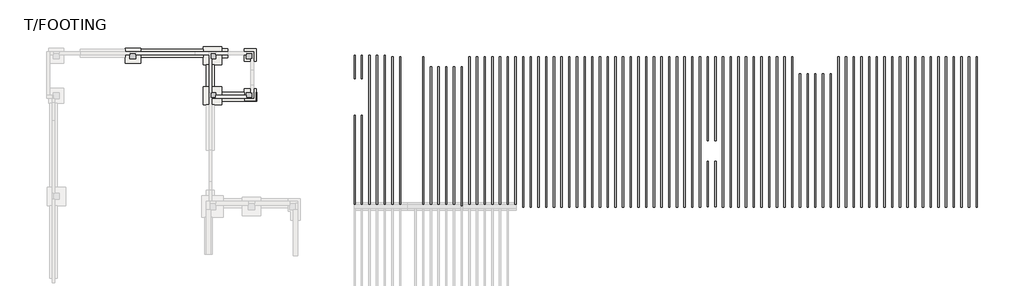
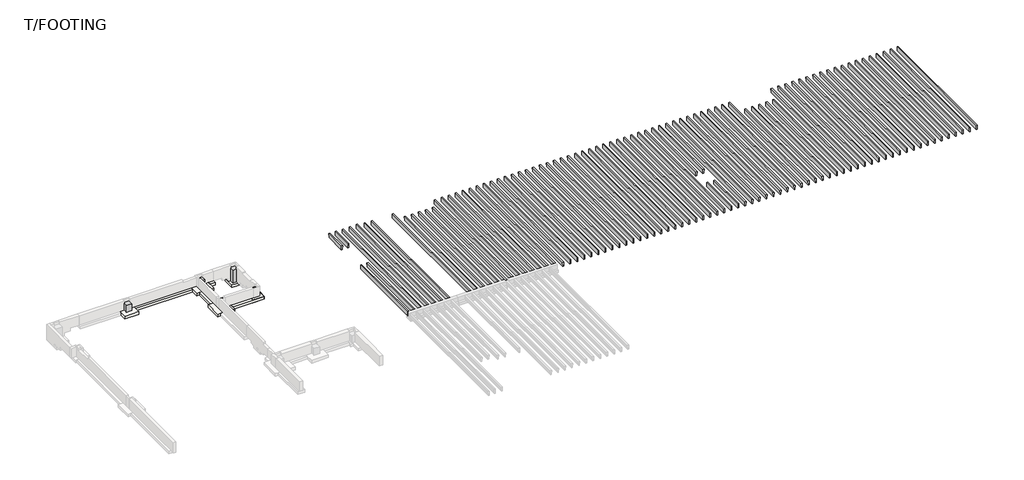
# One storey, part 3 of 3: 84 beams, 5 columns, 5 slabs, 4 footings.
"""IFC4 building model written with IfcOpenShell, lengths in millimetres."""

import ifcopenshell
import ifcopenshell.guid

model = None  # the IFC model being written
_history = None  # IfcOwnerHistory: only IFC2X3 demands one
_inside = {}  # id of a spatial element -> (the spatial element, [elements in it])
_under = {}  # id of a project, library or spatial element -> (it, [spatial elements below it])
_declared = {}  # id of a project -> (the project, [libraries it declares])
_typed = {}  # id of a type object -> (the type object, [elements of that type])
_made_of = {}  # id of a material, layer set ... -> (it, [elements and type objects made of it])


def new_model(schema):
    """Start an empty IFC model of exactly this schema.

    Asked for "IFC4X3", IfcOpenShell would pick the latest addendum, in which some entities
    have other attributes; the version numbers below select the first issue.
    IFC2X3 requires an IfcOwnerHistory on every rooted entity: one is made here for all.
    """
    global model, _history
    if schema == "IFC4X3":
        model = ifcopenshell.file(schema_version=(4, 3, 0, 0))
    else:
        model = ifcopenshell.file(schema=schema)
    _inside.clear()
    _under.clear()
    _declared.clear()
    _typed.clear()
    _made_of.clear()
    _history = None
    if model.schema == "IFC2X3":
        org = make("IfcOrganization", Name="unknown")
        user = make(
            "IfcPersonAndOrganization",
            ThePerson=make("IfcPerson", FamilyName="unknown"),
            TheOrganization=org,
        )
        app = make(
            "IfcApplication",
            ApplicationDeveloper=org,
            Version="unknown",
            ApplicationFullName="unknown",
            ApplicationIdentifier="unknown",
        )
        _history = make(
            "IfcOwnerHistory",
            OwningUser=user,
            OwningApplication=app,
            ChangeAction="ADDED",
            CreationDate=0,
        )
    return model


def make(cls, **values):
    """One entity of the class cls with the attributes given. An attribute that is None is left unset."""
    return model.create_entity(
        cls, **{name: value for name, value in values.items() if value is not None}
    )


def rooted(cls, **values):
    """An entity with a GlobalId (a new one), such as an element, a storey or a relation."""
    return make(cls, GlobalId=ifcopenshell.guid.new(), OwnerHistory=_history, **values)


def si_unit(unit_type, name, prefix=None):
    """IfcSIUnit, for example si_unit("LENGTHUNIT", "METRE", prefix="MILLI")."""
    return make("IfcSIUnit", UnitType=unit_type, Prefix=prefix, Name=name)


def assignment(units):
    """IfcUnitAssignment: the units of a project."""
    return None if units is None else make("IfcUnitAssignment", Units=units)


def point(xyz):
    """IfcCartesianPoint."""
    return None if xyz is None else make("IfcCartesianPoint", Coordinates=xyz)


def direction(xyz):
    """IfcDirection."""
    return None if xyz is None else make("IfcDirection", DirectionRatios=xyz)


def frame(location, z_axis=None, x_axis=None):
    """IfcAxis2Placement3D, a coordinate frame: its origin and axes. An axis left out is left unset."""
    return make(
        "IfcAxis2Placement3D",
        Location=point(location),
        Axis=direction(z_axis),
        RefDirection=direction(x_axis),
    )


def origin():
    """The frame at (0, 0, 0) with its axes left unset."""
    return frame((0.0, 0.0, 0.0))


def place(relative_to, where):
    """IfcLocalPlacement: puts the frame where relative to a parent placement (None: the world)."""
    return make(
        "IfcLocalPlacement", PlacementRelTo=relative_to, RelativePlacement=where
    )


def context(
    kind, dimensions, precision=None, world=None, true_north=None, identifier=None
):
    """IfcGeometricRepresentationContext, for example the 3D "Model" context."""
    return make(
        "IfcGeometricRepresentationContext",
        ContextIdentifier=identifier,
        ContextType=kind,
        CoordinateSpaceDimension=dimensions,
        Precision=precision,
        WorldCoordinateSystem=world,
        TrueNorth=true_north,
    )


def project(units=None, contexts=None):
    """IfcProject with its units and contexts."""
    return rooted(
        "IfcProject",
        Name="project",
        RepresentationContexts=contexts,
        UnitsInContext=assignment(units),
    )


def spatial(cls, under=None, at=None, **own):
    """A site, building, storey or space (cls), placed at a placement, below another one or the project."""
    s = rooted(cls, ObjectPlacement=at, **own)
    if under is not None:
        _under.setdefault(under.id(), (under, []))[1].append(s)
    return s


def polyline(points):
    """IfcPolyline through the points."""
    return make("IfcPolyline", Points=[point(p) for p in points])


def outline(outer, holes=None, kind="AREA"):
    """IfcArbitraryClosedProfileDef: a profile drawn as a closed curve; with holes, ...WithVoids."""
    if holes is None:
        return make("IfcArbitraryClosedProfileDef", ProfileType=kind, OuterCurve=outer)
    return make(
        "IfcArbitraryProfileDefWithVoids",
        ProfileType=kind,
        OuterCurve=outer,
        InnerCurves=holes,
    )


def extrude(swept, where, along, depth):
    """IfcExtrudedAreaSolid: the profile swept, set in the frame where, extruded along a direction by depth."""
    return make(
        "IfcExtrudedAreaSolid",
        SweptArea=swept,
        Position=where,
        ExtrudedDirection=direction(along),
        Depth=depth,
    )


def faces_of(points, faces, orient=None, outer=None):
    """IfcFace entities. A face is a list of loops; a loop is a list of indices into points, from 0.

    orient and outer hold one flag for each loop. By default every Orientation is true, the
    first loop of a face is its IfcFaceOuterBound and the others are IfcFaceBound.
    """
    made = []
    for i, loops in enumerate(faces):
        bounds = []
        for j, loop in enumerate(loops):
            is_outer = j == 0 if outer is None else outer[i][j]
            bounds.append(
                make(
                    "IfcFaceOuterBound" if is_outer else "IfcFaceBound",
                    Bound=make("IfcPolyLoop", Polygon=[points[k] for k in loop]),
                    Orientation=True if orient is None else orient[i][j],
                )
            )
        made.append(make("IfcFace", Bounds=bounds))
    return made


def faceted_brep(points, faces, orient=None, outer=None, voids=None):
    """IfcFacetedBrep: a solid bounded by flat faces; with voids (closed shells), ...WithVoids."""
    shared = [point(p) for p in points]
    hull = make("IfcClosedShell", CfsFaces=faces_of(shared, faces, orient, outer))
    if voids is None:
        return make("IfcFacetedBrep", Outer=hull)
    return make(
        "IfcFacetedBrepWithVoids",
        Outer=hull,
        Voids=[
            make(cls, CfsFaces=faces_of(shared, fs, o, b)) for cls, fs, o, b in voids
        ],
    )


def shape(context_of_items, identifier, shape_type, items):
    """IfcShapeRepresentation: the items that make up one representation, for example the "Body"."""
    return make(
        "IfcShapeRepresentation",
        ContextOfItems=context_of_items,
        RepresentationIdentifier=identifier,
        RepresentationType=shape_type,
        Items=items,
    )


def source(mapping_origin, context_of_items, identifier, shape_type, items):
    """IfcRepresentationMap: a shape defined once, which mapped items show again and again."""
    return make(
        "IfcRepresentationMap",
        MappingOrigin=mapping_origin,
        MappedRepresentation=shape(context_of_items, identifier, shape_type, items),
    )


def transform(
    local_origin,
    x_axis=None,
    y_axis=None,
    z_axis=None,
    scale=None,
    scale2=None,
    scale3=None,
    uniform=True,
):
    """IfcCartesianTransformationOperator3D, or its non-uniform kind. x_axis, y_axis, z_axis: its Axis1, 2, 3."""
    if uniform:
        return make(
            "IfcCartesianTransformationOperator3D",
            Axis1=direction(x_axis),
            Axis2=direction(y_axis),
            LocalOrigin=point(local_origin),
            Scale=scale,
            Axis3=direction(z_axis),
        )
    return make(
        "IfcCartesianTransformationOperator3DnonUniform",
        Axis1=direction(x_axis),
        Axis2=direction(y_axis),
        LocalOrigin=point(local_origin),
        Scale=scale,
        Axis3=direction(z_axis),
        Scale2=scale2,
        Scale3=scale3,
    )


def mapped(mapping_source, mapping_target):
    """IfcMappedItem: shows the shape of a source again, moved by a transform."""
    return make(
        "IfcMappedItem", MappingSource=mapping_source, MappingTarget=mapping_target
    )


def made_of(thing, what):
    """Note that an element or type object is made of a material, layer set ...; save() writes the relation."""
    if what is not None:
        _made_of.setdefault(what.id(), (what, []))[1].append(thing)
    return thing


def element(
    cls,
    number,
    at=None,
    inside=None,
    cuts=None,
    type_object=None,
    material=None,
    context=None,
    identifier="Body",
    shape_type=None,
    held_by="IfcProductDefinitionShape",
    body=None,
    shapes=None,
    **own,
):
    """One element of the class cls, such as IfcWall. Its Tag is "e" and its number.

    at: its placement. inside: the storey or other place that contains it. cuts: it is an
    opening in that element (IfcRelVoidsElement). A single representation is given by context,
    identifier, shape_type and body (its items); several are given by shapes. held_by: the class
    of the entity that holds the representations. save() writes the other relations.
    """
    e = rooted(cls, Tag="e%d" % number, ObjectPlacement=at, **own)
    if body is not None:
        shapes = [shape(context, identifier, shape_type, body)]
    if shapes is not None:
        e.Representation = make(held_by, Representations=shapes)
    if inside is not None:
        _inside.setdefault(inside.id(), (inside, []))[1].append(e)
    if cuts is not None:
        rooted(
            "IfcRelVoidsElement", RelatingBuildingElement=cuts, RelatedOpeningElement=e
        )
    if type_object is not None:
        _typed.setdefault(type_object.id(), (type_object, []))[1].append(e)
    return made_of(e, material)


def aggregate(whole, parts):
    """IfcRelAggregates: a whole, such as a stair, and the parts it consists of."""
    return rooted("IfcRelAggregates", RelatingObject=whole, RelatedObjects=parts)


def save(model, path):
    """Write the relations noted so far, then the file.

    IfcRelAggregates (storeys below a building ...), IfcRelContainedInSpatialStructure (elements
    in a storey), IfcRelDefinesByType, IfcRelAssociatesMaterial and IfcRelDeclares: one each for
    every whole, place, type object, material and project.
    """
    for whole, parts in _under.values():
        aggregate(whole, parts)
    for where, things in _inside.values():
        rooted(
            "IfcRelContainedInSpatialStructure",
            RelatedElements=things,
            RelatingStructure=where,
        )
    for kind, things in _typed.values():
        rooted("IfcRelDefinesByType", RelatedObjects=things, RelatingType=kind)
    for what, things in _made_of.values():
        rooted("IfcRelAssociatesMaterial", RelatedObjects=things, RelatingMaterial=what)
    for by, libraries in _declared.values():
        rooted("IfcRelDeclares", RelatingContext=by, RelatedDefinitions=libraries)
    model.write(path)


def precast_cone_shaped_beam_double_t_5f2c7775(model_context):
    return source(origin(), model_context, "Body", "SweptSolid", [
        extrude(outline(polyline([(50.8, -228.6), (-50.8, -228.6), (-63.5, 228.6), (63.5, 228.6), (50.8, -228.6)])), frame((-7353.3, 0.0, 0.0), z_axis=(1.0, 0.0, 0.0), x_axis=(0.0, 1.0, 0.0)), (0.0, 0.0, 1.0), 14693.9),
    ])


def precast_cone_shaped_beam_double_t_00600c4c(model_context):
    return source(origin(), model_context, "Body", "SweptSolid", [
        extrude(outline(polyline([(50.8, -228.6), (-50.8, -228.6), (-63.5, 228.6), (63.5, 228.6), (50.8, -228.6)])), frame((-7556.5, 0.0, 0.0), z_axis=(1.0, 0.0, 0.0), x_axis=(0.0, 1.0, 0.0)), (0.0, 0.0, 1.0), 14897.1),
    ])


def precast_cone_shaped_beam_double_t_e3fa137c(model_context):
    return source(origin(), model_context, "Body", "SweptSolid", [
        extrude(outline(polyline([(50.8, -228.6), (-50.8, -228.6), (-63.5, 228.6), (63.5, 228.6), (50.8, -228.6)])), frame((-4296.56875, 0.0, 0.0), z_axis=(1.0, 0.0, 0.0), x_axis=(0.0, 1.0, 0.0)), (0.0, 0.0, 1.0), 8318.5),
    ])


def precast_cone_shaped_beam_double_t_ce46092e(model_context):
    return source(origin(), model_context, "Body", "SweptSolid", [
        extrude(outline(polyline([(-50.8, -228.6), (-63.5, 228.6), (63.5, 228.6), (50.8, -228.6), (-50.8, -228.6)])), frame((-2302.66875, 0.0, 0.0), z_axis=(1.0, 0.0, 0.0), x_axis=(0.0, 1.0, 0.0)), (0.0, 0.0, 1.0), 4495.8),
    ])


def precast_cone_shaped_beam_double_t_099a914b(model_context):
    return source(origin(), model_context, "Body", "SweptSolid", [
        extrude(outline(polyline([(50.8, -228.6), (-50.8, -228.6), (-63.5, 228.6), (63.5, 228.6), (50.8, -228.6)])), frame((-6574.63125, 0.0, 0.0), z_axis=(1.0, 0.0, 0.0), x_axis=(0.0, 1.0, 0.0)), (0.0, 0.0, 1.0), 13208.0),
    ])


def precast_cone_shaped_beam_double_t_b8a3e37e(model_context):
    return source(origin(), model_context, "Body", "SweptSolid", [
        extrude(outline(polyline([(50.8, -228.6), (-50.8, -228.6), (-63.5, 228.6), (63.5, 228.6), (50.8, -228.6)])), frame((-6727.03125, 0.0, 0.0), z_axis=(1.0, 0.0, 0.0), x_axis=(0.0, 1.0, 0.0)), (0.0, 0.0, 1.0), 13716.0),
    ])


def precast_cone_shaped_beam_double_t_383d5be5(model_context):
    return source(origin(), model_context, "Body", "SweptSolid", [
        extrude(outline(polyline([(50.8, -228.6), (-50.8, -228.6), (-63.5, 228.6), (63.5, 228.6), (50.8, -228.6)])), frame((-6930.23125, 0.0, 0.0), z_axis=(1.0, 0.0, 0.0), x_axis=(0.0, 1.0, 0.0)), (0.0, 0.0, 1.0), 13919.2),
    ])


def precast_cone_shaped_beam_double_t_e38496ef(model_context):
    return source(origin(), model_context, "Body", "SweptSolid", [
        extrude(outline(polyline([(50.8, -228.6), (-50.8, -228.6), (-63.5, 228.6), (63.5, 228.6), (50.8, -228.6)])), frame((-4311.8111314, 0.0, 0.0), z_axis=(1.0, 0.0, 0.0), x_axis=(0.0, 1.0, 0.0)), (0.0, 0.0, 1.0), 8885.5597628),
    ])


def precast_cone_shaped_beam_double_t_7663fcfe(model_context):
    return source(origin(), model_context, "Body", "SweptSolid", [
        extrude(outline(polyline([(-50.8, -228.6), (-63.5, 228.6), (63.5, 228.6), (50.8, -228.6), (-50.8, -228.6)])), frame((-1119.0263686, 0.0, 0.0), z_axis=(1.0, 0.0, 0.0), x_axis=(0.0, 1.0, 0.0)), (0.0, 0.0, 1.0), 2347.5902372),
    ])


def precast_cone_shaped_beam_double_t_3d71fa44(model_context):
    return source(origin(), model_context, "Body", "SweptSolid", [
        extrude(outline(polyline([(50.8, -228.6), (-50.8, -228.6), (-63.5, 228.6), (63.5, 228.6), (50.8, -228.6)])), frame((-7353.3, 0.0, 0.0), z_axis=(1.0, 0.0, 0.0), x_axis=(0.0, 1.0, 0.0)), (0.0, 0.0, 1.0), 14859.0),
    ])


model = new_model("IFC4")

# Units and contexts
model_context = context("Model", 3, world=origin())
ifc_project = project(units=[si_unit("LENGTHUNIT", "METRE", prefix="MILLI")], contexts=[model_context])

# Site, building, storey
site = spatial("IfcSite", under=ifc_project)
building = spatial("IfcBuilding", under=site)
storey = spatial("IfcBuildingStorey", under=building, Name="T/FOOTING", Elevation=-1092.2)

# Beams
placement = place(None, origin())
precast_cone_shaped_beam_double_t_shape = precast_cone_shaped_beam_double_t_5f2c7775(model_context)
element("IfcBeam", 1, ObjectType="Precast-Cone Shaped Beam : DOUBLE_T", at=placement, inside=storey, context=model_context, shape_type="MappedRepresentation", body=[
    mapped(precast_cone_shaped_beam_double_t_shape, transform((-28033.5909443, 5341.6768471, -279.4), x_axis=(0.0, 1.0, 0.0), y_axis=(-1.0, 0.0, 0.0), z_axis=(0.0, 0.0, 1.0))),
])
element("IfcBeam", 2, ObjectType="Precast-Cone Shaped Beam : DOUBLE_T", at=placement, inside=storey, context=model_context, shape_type="MappedRepresentation", body=[
    mapped(precast_cone_shaped_beam_double_t_shape, transform((-23461.5909443, 5341.6768471, -279.4), x_axis=(0.0, 1.0, 0.0), y_axis=(-1.0, 0.0, 0.0), z_axis=(0.0, 0.0, 1.0))),
])
element("IfcBeam", 3, ObjectType="Precast-Cone Shaped Beam : DOUBLE_T", at=placement, inside=storey, context=model_context, shape_type="MappedRepresentation", body=[
    mapped(precast_cone_shaped_beam_double_t_shape, transform((-22699.5909443, 5341.6768471, -279.4), x_axis=(0.0, 1.0, 0.0), y_axis=(-1.0, 0.0, 0.0), z_axis=(0.0, 0.0, 1.0))),
])
element("IfcBeam", 4, ObjectType="Precast-Cone Shaped Beam : DOUBLE_T", at=placement, inside=storey, context=model_context, shape_type="MappedRepresentation", body=[
    mapped(precast_cone_shaped_beam_double_t_shape, transform((-21940.4905844, 5341.6768471, -279.4), x_axis=(0.0, 1.0, 0.0), y_axis=(-1.0, 0.0, 0.0), z_axis=(0.0, 0.0, 1.0))),
])
element("IfcBeam", 5, ObjectType="Precast-Cone Shaped Beam : DOUBLE_T", at=placement, inside=storey, context=model_context, shape_type="MappedRepresentation", body=[
    mapped(precast_cone_shaped_beam_double_t_shape, transform((-21179.5348789, 5341.6768471, -279.4), x_axis=(0.0, 1.0, 0.0), y_axis=(-1.0, 0.0, 0.0), z_axis=(0.0, 0.0, 1.0))),
])
element("IfcBeam", 6, ObjectType="Precast-Cone Shaped Beam : DOUBLE_T", at=placement, inside=storey, context=model_context, shape_type="MappedRepresentation", body=[
    mapped(precast_cone_shaped_beam_double_t_shape, transform((-20417.5348789, 5341.6768471, -279.4), x_axis=(0.0, 1.0, 0.0), y_axis=(-1.0, 0.0, 0.0), z_axis=(0.0, 0.0, 1.0))),
])
element("IfcBeam", 7, ObjectType="Precast-Cone Shaped Beam : DOUBLE_T", at=placement, inside=storey, context=model_context, shape_type="MappedRepresentation", body=[
    mapped(precast_cone_shaped_beam_double_t_shape, transform((-19655.5348789, 5341.6768471, -279.4), x_axis=(0.0, 1.0, 0.0), y_axis=(-1.0, 0.0, 0.0), z_axis=(0.0, 0.0, 1.0))),
])
element("IfcBeam", 8, ObjectType="Precast-Cone Shaped Beam : DOUBLE_T", at=placement, inside=storey, context=model_context, shape_type="MappedRepresentation", body=[
    mapped(precast_cone_shaped_beam_double_t_shape, transform((-18893.5348789, 5341.6768471, -279.4), x_axis=(0.0, 1.0, 0.0), y_axis=(-1.0, 0.0, 0.0), z_axis=(0.0, 0.0, 1.0))),
])
element("IfcBeam", 9, ObjectType="Precast-Cone Shaped Beam : DOUBLE_T", at=placement, inside=storey, context=model_context, shape_type="MappedRepresentation", body=[
    mapped(precast_cone_shaped_beam_double_t_shape, transform((-30319.5909443, 5341.6768471, -279.4), x_axis=(0.0, 1.0, 0.0), y_axis=(-1.0, 0.0, 0.0), z_axis=(0.0, 0.0, 1.0))),
])
element("IfcBeam", 10, ObjectType="Precast-Cone Shaped Beam : DOUBLE_T", at=placement, inside=storey, context=model_context, shape_type="MappedRepresentation", body=[
    mapped(precast_cone_shaped_beam_double_t_shape, transform((-31081.5909443, 5341.6768471, -279.4), x_axis=(0.0, 1.0, 0.0), y_axis=(-1.0, 0.0, 0.0), z_axis=(0.0, 0.0, 1.0))),
])
precast_cone_shaped_beam_double_t_2_shape = precast_cone_shaped_beam_double_t_00600c4c(model_context)
element("IfcBeam", 11, ObjectType="Precast-Cone Shaped Beam : DOUBLE_T", at=placement, inside=storey, context=model_context, shape_type="MappedRepresentation", body=[
    mapped(precast_cone_shaped_beam_double_t_2_shape, transform((-18131.5348789, 5341.6768471, -279.4), x_axis=(0.0, 1.0, 0.0), y_axis=(-1.0, 0.0, 0.0), z_axis=(0.0, 0.0, 1.0))),
])
element("IfcBeam", 12, ObjectType="Precast-Cone Shaped Beam : DOUBLE_T", at=placement, inside=storey, context=model_context, shape_type="MappedRepresentation", body=[
    mapped(precast_cone_shaped_beam_double_t_2_shape, transform((-17369.5348789, 5341.6768471, -279.4), x_axis=(0.0, 1.0, 0.0), y_axis=(-1.0, 0.0, 0.0), z_axis=(0.0, 0.0, 1.0))),
])
element("IfcBeam", 13, ObjectType="Precast-Cone Shaped Beam : DOUBLE_T", at=placement, inside=storey, context=model_context, shape_type="MappedRepresentation", body=[
    mapped(precast_cone_shaped_beam_double_t_2_shape, transform((-16607.5348789, 5341.6768471, -279.4), x_axis=(0.0, 1.0, 0.0), y_axis=(-1.0, 0.0, 0.0), z_axis=(0.0, 0.0, 1.0))),
])
element("IfcBeam", 14, ObjectType="Precast-Cone Shaped Beam : DOUBLE_T", at=placement, inside=storey, context=model_context, shape_type="MappedRepresentation", body=[
    mapped(precast_cone_shaped_beam_double_t_2_shape, transform((-15845.5348789, 5341.6768471, -279.4), x_axis=(0.0, 1.0, 0.0), y_axis=(-1.0, 0.0, 0.0), z_axis=(0.0, 0.0, 1.0))),
])
element("IfcBeam", 15, ObjectType="Precast-Cone Shaped Beam : DOUBLE_T", at=placement, inside=storey, context=model_context, shape_type="MappedRepresentation", body=[
    mapped(precast_cone_shaped_beam_double_t_2_shape, transform((-15083.5348789, 5341.6768471, -279.4), x_axis=(0.0, 1.0, 0.0), y_axis=(-1.0, 0.0, 0.0), z_axis=(0.0, 0.0, 1.0))),
])
element("IfcBeam", 16, ObjectType="Precast-Cone Shaped Beam : DOUBLE_T", at=placement, inside=storey, context=model_context, shape_type="MappedRepresentation", body=[
    mapped(precast_cone_shaped_beam_double_t_2_shape, transform((-14321.5348789, 5341.6768471, -279.4), x_axis=(0.0, 1.0, 0.0), y_axis=(-1.0, 0.0, 0.0), z_axis=(0.0, 0.0, 1.0))),
])
element("IfcBeam", 17, ObjectType="Precast-Cone Shaped Beam : DOUBLE_T", at=placement, inside=storey, context=model_context, shape_type="MappedRepresentation", body=[
    mapped(precast_cone_shaped_beam_double_t_2_shape, transform((-13559.5348789, 5341.6768471, -279.4), x_axis=(0.0, 1.0, 0.0), y_axis=(-1.0, 0.0, 0.0), z_axis=(0.0, 0.0, 1.0))),
])
element("IfcBeam", 18, ObjectType="Precast-Cone Shaped Beam : DOUBLE_T", at=placement, inside=storey, context=model_context, shape_type="MappedRepresentation", body=[
    mapped(precast_cone_shaped_beam_double_t_2_shape, transform((-12797.5348789, 5341.6768471, -279.4), x_axis=(0.0, 1.0, 0.0), y_axis=(-1.0, 0.0, 0.0), z_axis=(0.0, 0.0, 1.0))),
])
element("IfcBeam", 19, ObjectType="Precast-Cone Shaped Beam : DOUBLE_T", at=placement, inside=storey, context=model_context, shape_type="MappedRepresentation", body=[
    mapped(precast_cone_shaped_beam_double_t_2_shape, transform((-12035.5348789, 5341.6768471, -279.4), x_axis=(0.0, 1.0, 0.0), y_axis=(-1.0, 0.0, 0.0), z_axis=(0.0, 0.0, 1.0))),
])
element("IfcBeam", 20, ObjectType="Precast-Cone Shaped Beam : DOUBLE_T", at=placement, inside=storey, context=model_context, shape_type="MappedRepresentation", body=[
    mapped(precast_cone_shaped_beam_double_t_2_shape, transform((-11273.5348789, 5341.6768471, -279.4), x_axis=(0.0, 1.0, 0.0), y_axis=(-1.0, 0.0, 0.0), z_axis=(0.0, 0.0, 1.0))),
])
element("IfcBeam", 21, ObjectType="Precast-Cone Shaped Beam : DOUBLE_T", at=placement, inside=storey, context=model_context, shape_type="MappedRepresentation", body=[
    mapped(precast_cone_shaped_beam_double_t_2_shape, transform((-10511.5348789, 5341.6768471, -279.4), x_axis=(0.0, 1.0, 0.0), y_axis=(-1.0, 0.0, 0.0), z_axis=(0.0, 0.0, 1.0))),
])
element("IfcBeam", 22, ObjectType="Precast-Cone Shaped Beam : DOUBLE_T", at=placement, inside=storey, context=model_context, shape_type="MappedRepresentation", body=[
    mapped(precast_cone_shaped_beam_double_t_2_shape, transform((-9749.5348789, 5341.6768471, -279.4), x_axis=(0.0, 1.0, 0.0), y_axis=(-1.0, 0.0, 0.0), z_axis=(0.0, 0.0, 1.0))),
])
element("IfcBeam", 23, ObjectType="Precast-Cone Shaped Beam : DOUBLE_T", at=placement, inside=storey, context=model_context, shape_type="MappedRepresentation", body=[
    mapped(precast_cone_shaped_beam_double_t_2_shape, transform((-8987.5348789, 5341.6768471, -279.4), x_axis=(0.0, 1.0, 0.0), y_axis=(-1.0, 0.0, 0.0), z_axis=(0.0, 0.0, 1.0))),
])
element("IfcBeam", 24, ObjectType="Precast-Cone Shaped Beam : DOUBLE_T", at=placement, inside=storey, context=model_context, shape_type="MappedRepresentation", body=[
    mapped(precast_cone_shaped_beam_double_t_2_shape, transform((-8225.5348789, 5341.6768471, -279.4), x_axis=(0.0, 1.0, 0.0), y_axis=(-1.0, 0.0, 0.0), z_axis=(0.0, 0.0, 1.0))),
])
element("IfcBeam", 25, ObjectType="Precast-Cone Shaped Beam : DOUBLE_T", at=placement, inside=storey, context=model_context, shape_type="MappedRepresentation", body=[
    mapped(precast_cone_shaped_beam_double_t_2_shape, transform((-7463.5348789, 5341.6768471, -279.4), x_axis=(0.0, 1.0, 0.0), y_axis=(-1.0, 0.0, 0.0), z_axis=(0.0, 0.0, 1.0))),
])
element("IfcBeam", 26, ObjectType="Precast-Cone Shaped Beam : DOUBLE_T", at=placement, inside=storey, context=model_context, shape_type="MappedRepresentation", body=[
    mapped(precast_cone_shaped_beam_double_t_2_shape, transform((-6701.5348789, 5341.6768471, -279.4), x_axis=(0.0, 1.0, 0.0), y_axis=(-1.0, 0.0, 0.0), z_axis=(0.0, 0.0, 1.0))),
])
element("IfcBeam", 27, ObjectType="Precast-Cone Shaped Beam : DOUBLE_T", at=placement, inside=storey, context=model_context, shape_type="MappedRepresentation", body=[
    mapped(precast_cone_shaped_beam_double_t_2_shape, transform((-5939.5348789, 5341.6768471, -279.4), x_axis=(0.0, 1.0, 0.0), y_axis=(-1.0, 0.0, 0.0), z_axis=(0.0, 0.0, 1.0))),
])
element("IfcBeam", 28, ObjectType="Precast-Cone Shaped Beam : DOUBLE_T", at=placement, inside=storey, context=model_context, shape_type="MappedRepresentation", body=[
    mapped(precast_cone_shaped_beam_double_t_2_shape, transform((-5177.5348789, 5341.6768471, -279.4), x_axis=(0.0, 1.0, 0.0), y_axis=(-1.0, 0.0, 0.0), z_axis=(0.0, 0.0, 1.0))),
])
element("IfcBeam", 29, ObjectType="Precast-Cone Shaped Beam : DOUBLE_T", at=placement, inside=storey, context=model_context, shape_type="MappedRepresentation", body=[
    mapped(precast_cone_shaped_beam_double_t_2_shape, transform((-4415.5348789, 5341.6768471, -279.4), x_axis=(0.0, 1.0, 0.0), y_axis=(-1.0, 0.0, 0.0), z_axis=(0.0, 0.0, 1.0))),
])
element("IfcBeam", 30, ObjectType="Precast-Cone Shaped Beam : DOUBLE_T", at=placement, inside=storey, context=model_context, shape_type="MappedRepresentation", body=[
    mapped(precast_cone_shaped_beam_double_t_2_shape, transform((-3653.5348789, 5341.6768471, -279.4), x_axis=(0.0, 1.0, 0.0), y_axis=(-1.0, 0.0, 0.0), z_axis=(0.0, 0.0, 1.0))),
])
element("IfcBeam", 31, ObjectType="Precast-Cone Shaped Beam : DOUBLE_T", at=placement, inside=storey, context=model_context, shape_type="MappedRepresentation", body=[
    mapped(precast_cone_shaped_beam_double_t_2_shape, transform((-2891.5348789, 5341.6768471, -279.4), x_axis=(0.0, 1.0, 0.0), y_axis=(-1.0, 0.0, 0.0), z_axis=(0.0, 0.0, 1.0))),
])
element("IfcBeam", 32, ObjectType="Precast-Cone Shaped Beam : DOUBLE_T", at=placement, inside=storey, context=model_context, shape_type="MappedRepresentation", body=[
    mapped(precast_cone_shaped_beam_double_t_2_shape, transform((-2129.5348789, 5341.6768471, -279.4), x_axis=(0.0, 1.0, 0.0), y_axis=(-1.0, 0.0, 0.0), z_axis=(0.0, 0.0, 1.0))),
])
element("IfcBeam", 33, ObjectType="Precast-Cone Shaped Beam : DOUBLE_T", at=placement, inside=storey, context=model_context, shape_type="MappedRepresentation", body=[
    mapped(precast_cone_shaped_beam_double_t_2_shape, transform((-1367.5348789, 5341.6768471, -279.4), x_axis=(0.0, 1.0, 0.0), y_axis=(-1.0, 0.0, 0.0), z_axis=(0.0, 0.0, 1.0))),
])
element("IfcBeam", 34, ObjectType="Precast-Cone Shaped Beam : DOUBLE_T", at=placement, inside=storey, context=model_context, shape_type="MappedRepresentation", body=[
    mapped(precast_cone_shaped_beam_double_t_2_shape, transform((-605.5348789, 5341.6768471, -279.4), x_axis=(0.0, 1.0, 0.0), y_axis=(-1.0, 0.0, 0.0), z_axis=(0.0, 0.0, 1.0))),
])
element("IfcBeam", 35, ObjectType="Precast-Cone Shaped Beam : DOUBLE_T", at=placement, inside=storey, context=model_context, shape_type="MappedRepresentation", body=[
    mapped(precast_cone_shaped_beam_double_t_2_shape, transform((1680.4651211, 5341.6768471, -279.4), x_axis=(0.0, 1.0, 0.0), y_axis=(-1.0, 0.0, 0.0), z_axis=(0.0, 0.0, 1.0))),
])
element("IfcBeam", 36, ObjectType="Precast-Cone Shaped Beam : DOUBLE_T", at=placement, inside=storey, context=model_context, shape_type="MappedRepresentation", body=[
    mapped(precast_cone_shaped_beam_double_t_2_shape, transform((2442.4651211, 5341.6768471, -279.4), x_axis=(0.0, 1.0, 0.0), y_axis=(-1.0, 0.0, 0.0), z_axis=(0.0, 0.0, 1.0))),
])
element("IfcBeam", 37, ObjectType="Precast-Cone Shaped Beam : DOUBLE_T", at=placement, inside=storey, context=model_context, shape_type="MappedRepresentation", body=[
    mapped(precast_cone_shaped_beam_double_t_2_shape, transform((3204.4651211, 5341.6768471, -279.4), x_axis=(0.0, 1.0, 0.0), y_axis=(-1.0, 0.0, 0.0), z_axis=(0.0, 0.0, 1.0))),
])
element("IfcBeam", 38, ObjectType="Precast-Cone Shaped Beam : DOUBLE_T", at=placement, inside=storey, context=model_context, shape_type="MappedRepresentation", body=[
    mapped(precast_cone_shaped_beam_double_t_2_shape, transform((3966.4651211, 5341.6768471, -279.4), x_axis=(0.0, 1.0, 0.0), y_axis=(-1.0, 0.0, 0.0), z_axis=(0.0, 0.0, 1.0))),
])
element("IfcBeam", 39, ObjectType="Precast-Cone Shaped Beam : DOUBLE_T", at=placement, inside=storey, context=model_context, shape_type="MappedRepresentation", body=[
    mapped(precast_cone_shaped_beam_double_t_2_shape, transform((4728.4651211, 5341.6768471, -279.4), x_axis=(0.0, 1.0, 0.0), y_axis=(-1.0, 0.0, 0.0), z_axis=(0.0, 0.0, 1.0))),
])
element("IfcBeam", 40, ObjectType="Precast-Cone Shaped Beam : DOUBLE_T", at=placement, inside=storey, context=model_context, shape_type="MappedRepresentation", body=[
    mapped(precast_cone_shaped_beam_double_t_2_shape, transform((5490.4651211, 5341.6768471, -279.4), x_axis=(0.0, 1.0, 0.0), y_axis=(-1.0, 0.0, 0.0), z_axis=(0.0, 0.0, 1.0))),
])
element("IfcBeam", 41, ObjectType="Precast-Cone Shaped Beam : DOUBLE_T", at=placement, inside=storey, context=model_context, shape_type="MappedRepresentation", body=[
    mapped(precast_cone_shaped_beam_double_t_2_shape, transform((6252.4651211, 5341.6768471, -279.4), x_axis=(0.0, 1.0, 0.0), y_axis=(-1.0, 0.0, 0.0), z_axis=(0.0, 0.0, 1.0))),
])
element("IfcBeam", 42, ObjectType="Precast-Cone Shaped Beam : DOUBLE_T", at=placement, inside=storey, context=model_context, shape_type="MappedRepresentation", body=[
    mapped(precast_cone_shaped_beam_double_t_2_shape, transform((7014.4651211, 5341.6768471, -279.4), x_axis=(0.0, 1.0, 0.0), y_axis=(-1.0, 0.0, 0.0), z_axis=(0.0, 0.0, 1.0))),
])
element("IfcBeam", 43, ObjectType="Precast-Cone Shaped Beam : DOUBLE_T", at=placement, inside=storey, context=model_context, shape_type="MappedRepresentation", body=[
    mapped(precast_cone_shaped_beam_double_t_2_shape, transform((7776.4651211, 5341.6768471, -279.4), x_axis=(0.0, 1.0, 0.0), y_axis=(-1.0, 0.0, 0.0), z_axis=(0.0, 0.0, 1.0))),
])
element("IfcBeam", 44, ObjectType="Precast-Cone Shaped Beam : DOUBLE_T", at=placement, inside=storey, context=model_context, shape_type="MappedRepresentation", body=[
    mapped(precast_cone_shaped_beam_double_t_2_shape, transform((8538.4651211, 5341.6768471, -279.4), x_axis=(0.0, 1.0, 0.0), y_axis=(-1.0, 0.0, 0.0), z_axis=(0.0, 0.0, 1.0))),
])
element("IfcBeam", 45, ObjectType="Precast-Cone Shaped Beam : DOUBLE_T", at=placement, inside=storey, context=model_context, shape_type="MappedRepresentation", body=[
    mapped(precast_cone_shaped_beam_double_t_2_shape, transform((13110.4651211, 5341.6768471, -279.4), x_axis=(0.0, 1.0, 0.0), y_axis=(-1.0, 0.0, 0.0), z_axis=(0.0, 0.0, 1.0))),
])
element("IfcBeam", 46, ObjectType="Precast-Cone Shaped Beam : DOUBLE_T", at=placement, inside=storey, context=model_context, shape_type="MappedRepresentation", body=[
    mapped(precast_cone_shaped_beam_double_t_2_shape, transform((13872.4651211, 5341.6768471, -279.4), x_axis=(0.0, 1.0, 0.0), y_axis=(-1.0, 0.0, 0.0), z_axis=(0.0, 0.0, 1.0))),
])
element("IfcBeam", 47, ObjectType="Precast-Cone Shaped Beam : DOUBLE_T", at=placement, inside=storey, context=model_context, shape_type="MappedRepresentation", body=[
    mapped(precast_cone_shaped_beam_double_t_2_shape, transform((14634.4651211, 5341.6768471, -279.4), x_axis=(0.0, 1.0, 0.0), y_axis=(-1.0, 0.0, 0.0), z_axis=(0.0, 0.0, 1.0))),
])
element("IfcBeam", 48, ObjectType="Precast-Cone Shaped Beam : DOUBLE_T", at=placement, inside=storey, context=model_context, shape_type="MappedRepresentation", body=[
    mapped(precast_cone_shaped_beam_double_t_2_shape, transform((15396.4651211, 5341.6768471, -279.4), x_axis=(0.0, 1.0, 0.0), y_axis=(-1.0, 0.0, 0.0), z_axis=(0.0, 0.0, 1.0))),
])
element("IfcBeam", 49, ObjectType="Precast-Cone Shaped Beam : DOUBLE_T", at=placement, inside=storey, context=model_context, shape_type="MappedRepresentation", body=[
    mapped(precast_cone_shaped_beam_double_t_2_shape, transform((16158.4651211, 5341.6768471, -279.4), x_axis=(0.0, 1.0, 0.0), y_axis=(-1.0, 0.0, 0.0), z_axis=(0.0, 0.0, 1.0))),
])
element("IfcBeam", 50, ObjectType="Precast-Cone Shaped Beam : DOUBLE_T", at=placement, inside=storey, context=model_context, shape_type="MappedRepresentation", body=[
    mapped(precast_cone_shaped_beam_double_t_2_shape, transform((16920.4651211, 5341.6768471, -279.4), x_axis=(0.0, 1.0, 0.0), y_axis=(-1.0, 0.0, 0.0), z_axis=(0.0, 0.0, 1.0))),
])
element("IfcBeam", 51, ObjectType="Precast-Cone Shaped Beam : DOUBLE_T", at=placement, inside=storey, context=model_context, shape_type="MappedRepresentation", body=[
    mapped(precast_cone_shaped_beam_double_t_2_shape, transform((17682.4651211, 5341.6768471, -279.4), x_axis=(0.0, 1.0, 0.0), y_axis=(-1.0, 0.0, 0.0), z_axis=(0.0, 0.0, 1.0))),
])
element("IfcBeam", 52, ObjectType="Precast-Cone Shaped Beam : DOUBLE_T", at=placement, inside=storey, context=model_context, shape_type="MappedRepresentation", body=[
    mapped(precast_cone_shaped_beam_double_t_2_shape, transform((18444.4651211, 5341.6768471, -279.4), x_axis=(0.0, 1.0, 0.0), y_axis=(-1.0, 0.0, 0.0), z_axis=(0.0, 0.0, 1.0))),
])
element("IfcBeam", 53, ObjectType="Precast-Cone Shaped Beam : DOUBLE_T", at=placement, inside=storey, context=model_context, shape_type="MappedRepresentation", body=[
    mapped(precast_cone_shaped_beam_double_t_2_shape, transform((19206.4651211, 5341.6768471, -279.4), x_axis=(0.0, 1.0, 0.0), y_axis=(-1.0, 0.0, 0.0), z_axis=(0.0, 0.0, 1.0))),
])
element("IfcBeam", 54, ObjectType="Precast-Cone Shaped Beam : DOUBLE_T", at=placement, inside=storey, context=model_context, shape_type="MappedRepresentation", body=[
    mapped(precast_cone_shaped_beam_double_t_2_shape, transform((19968.4651211, 5341.6768471, -279.4), x_axis=(0.0, 1.0, 0.0), y_axis=(-1.0, 0.0, 0.0), z_axis=(0.0, 0.0, 1.0))),
])
element("IfcBeam", 55, ObjectType="Precast-Cone Shaped Beam : DOUBLE_T", at=placement, inside=storey, context=model_context, shape_type="MappedRepresentation", body=[
    mapped(precast_cone_shaped_beam_double_t_2_shape, transform((20730.4651211, 5341.6768471, -279.4), x_axis=(0.0, 1.0, 0.0), y_axis=(-1.0, 0.0, 0.0), z_axis=(0.0, 0.0, 1.0))),
])
element("IfcBeam", 56, ObjectType="Precast-Cone Shaped Beam : DOUBLE_T", at=placement, inside=storey, context=model_context, shape_type="MappedRepresentation", body=[
    mapped(precast_cone_shaped_beam_double_t_2_shape, transform((21492.4651211, 5341.6768471, -279.4), x_axis=(0.0, 1.0, 0.0), y_axis=(-1.0, 0.0, 0.0), z_axis=(0.0, 0.0, 1.0))),
])
element("IfcBeam", 57, ObjectType="Precast-Cone Shaped Beam : DOUBLE_T", at=placement, inside=storey, context=model_context, shape_type="MappedRepresentation", body=[
    mapped(precast_cone_shaped_beam_double_t_2_shape, transform((22254.4651211, 5341.6768471, -279.4), x_axis=(0.0, 1.0, 0.0), y_axis=(-1.0, 0.0, 0.0), z_axis=(0.0, 0.0, 1.0))),
])
element("IfcBeam", 58, ObjectType="Precast-Cone Shaped Beam : DOUBLE_T", at=placement, inside=storey, context=model_context, shape_type="MappedRepresentation", body=[
    mapped(precast_cone_shaped_beam_double_t_2_shape, transform((23016.4651211, 5341.6768471, -279.4), x_axis=(0.0, 1.0, 0.0), y_axis=(-1.0, 0.0, 0.0), z_axis=(0.0, 0.0, 1.0))),
])
element("IfcBeam", 59, ObjectType="Precast-Cone Shaped Beam : DOUBLE_T", at=placement, inside=storey, context=model_context, shape_type="MappedRepresentation", body=[
    mapped(precast_cone_shaped_beam_double_t_2_shape, transform((23778.4651211, 5341.6768471, -279.4), x_axis=(0.0, 1.0, 0.0), y_axis=(-1.0, 0.0, 0.0), z_axis=(0.0, 0.0, 1.0))),
])
element("IfcBeam", 60, ObjectType="Precast-Cone Shaped Beam : DOUBLE_T", at=placement, inside=storey, context=model_context, shape_type="MappedRepresentation", body=[
    mapped(precast_cone_shaped_beam_double_t_2_shape, transform((24540.4651211, 5341.6768471, -279.4), x_axis=(0.0, 1.0, 0.0), y_axis=(-1.0, 0.0, 0.0), z_axis=(0.0, 0.0, 1.0))),
])
element("IfcBeam", 61, ObjectType="Precast-Cone Shaped Beam : DOUBLE_T", at=placement, inside=storey, context=model_context, shape_type="MappedRepresentation", body=[
    mapped(precast_cone_shaped_beam_double_t_2_shape, transform((25302.4651211, 5341.6768471, -279.4), x_axis=(0.0, 1.0, 0.0), y_axis=(-1.0, 0.0, 0.0), z_axis=(0.0, 0.0, 1.0))),
])
element("IfcBeam", 62, ObjectType="Precast-Cone Shaped Beam : DOUBLE_T", at=placement, inside=storey, context=model_context, shape_type="MappedRepresentation", body=[
    mapped(precast_cone_shaped_beam_double_t_2_shape, transform((26064.4651211, 5341.6768471, -279.4), x_axis=(0.0, 1.0, 0.0), y_axis=(-1.0, 0.0, 0.0), z_axis=(0.0, 0.0, 1.0))),
])
element("IfcBeam", 63, ObjectType="Precast-Cone Shaped Beam : DOUBLE_T", at=placement, inside=storey, context=model_context, shape_type="MappedRepresentation", body=[
    mapped(precast_cone_shaped_beam_double_t_2_shape, transform((26826.4651211, 5341.6768471, -279.4), x_axis=(0.0, 1.0, 0.0), y_axis=(-1.0, 0.0, 0.0), z_axis=(0.0, 0.0, 1.0))),
])
precast_cone_shaped_beam_double_t_3_shape = precast_cone_shaped_beam_double_t_e3fa137c(model_context)
element("IfcBeam", 64, ObjectType="Precast-Cone Shaped Beam : DOUBLE_T", at=placement, inside=storey, context=model_context, shape_type="MappedRepresentation", body=[
    mapped(precast_cone_shaped_beam_double_t_3_shape, transform((156.4651211, 8660.3455971, -279.4), x_axis=(0.0, 1.0, 0.0), y_axis=(-1.0, 0.0, 0.0), z_axis=(0.0, 0.0, 1.0))),
])
element("IfcBeam", 65, ObjectType="Precast-Cone Shaped Beam : DOUBLE_T", at=placement, inside=storey, context=model_context, shape_type="MappedRepresentation", body=[
    mapped(precast_cone_shaped_beam_double_t_3_shape, transform((918.4651211, 8660.3455971, -279.4), x_axis=(0.0, 1.0, 0.0), y_axis=(-1.0, 0.0, 0.0), z_axis=(0.0, 0.0, 1.0))),
])
precast_cone_shaped_beam_double_t_4_shape = precast_cone_shaped_beam_double_t_ce46092e(model_context)
element("IfcBeam", 66, ObjectType="Precast-Cone Shaped Beam : DOUBLE_T", at=placement, inside=storey, context=model_context, shape_type="MappedRepresentation", body=[
    mapped(precast_cone_shaped_beam_double_t_4_shape, transform((156.4651211, 29.1080971, -279.4), x_axis=(0.0, -1.0, 0.0), y_axis=(1.0, 0.0, 0.0), z_axis=(0.0, 0.0, 1.0))),
])
element("IfcBeam", 67, ObjectType="Precast-Cone Shaped Beam : DOUBLE_T", at=placement, inside=storey, context=model_context, shape_type="MappedRepresentation", body=[
    mapped(precast_cone_shaped_beam_double_t_4_shape, transform((918.4651211, 29.1080971, -279.4), x_axis=(0.0, -1.0, 0.0), y_axis=(1.0, 0.0, 0.0), z_axis=(0.0, 0.0, 1.0))),
])
precast_cone_shaped_beam_double_t_5_shape = precast_cone_shaped_beam_double_t_099a914b(model_context)
element("IfcBeam", 68, ObjectType="Precast-Cone Shaped Beam : DOUBLE_T", at=placement, inside=storey, context=model_context, shape_type="MappedRepresentation", body=[
    mapped(precast_cone_shaped_beam_double_t_5_shape, transform((9300.4651211, 4359.8080971, -279.4), x_axis=(0.0, 1.0, 0.0), y_axis=(-1.0, 0.0, 0.0), z_axis=(0.0, 0.0, 1.0))),
])
element("IfcBeam", 69, ObjectType="Precast-Cone Shaped Beam : DOUBLE_T", at=placement, inside=storey, context=model_context, shape_type="MappedRepresentation", body=[
    mapped(precast_cone_shaped_beam_double_t_5_shape, transform((10062.4651211, 4359.8080971, -279.4), x_axis=(0.0, 1.0, 0.0), y_axis=(-1.0, 0.0, 0.0), z_axis=(0.0, 0.0, 1.0))),
])
element("IfcBeam", 70, ObjectType="Precast-Cone Shaped Beam : DOUBLE_T", at=placement, inside=storey, context=model_context, shape_type="MappedRepresentation", body=[
    mapped(precast_cone_shaped_beam_double_t_5_shape, transform((10824.4651211, 4359.8080971, -279.4), x_axis=(0.0, 1.0, 0.0), y_axis=(-1.0, 0.0, 0.0), z_axis=(0.0, 0.0, 1.0))),
])
element("IfcBeam", 71, ObjectType="Precast-Cone Shaped Beam : DOUBLE_T", at=placement, inside=storey, context=model_context, shape_type="MappedRepresentation", body=[
    mapped(precast_cone_shaped_beam_double_t_5_shape, transform((11586.4651211, 4359.8080971, -279.4), x_axis=(0.0, 1.0, 0.0), y_axis=(-1.0, 0.0, 0.0), z_axis=(0.0, 0.0, 1.0))),
])
element("IfcBeam", 72, ObjectType="Precast-Cone Shaped Beam : DOUBLE_T", at=placement, inside=storey, context=model_context, shape_type="MappedRepresentation", body=[
    mapped(precast_cone_shaped_beam_double_t_5_shape, transform((12348.4651211, 4359.8080971, -279.4), x_axis=(0.0, 1.0, 0.0), y_axis=(-1.0, 0.0, 0.0), z_axis=(0.0, 0.0, 1.0))),
])
precast_cone_shaped_beam_double_t_6_shape = precast_cone_shaped_beam_double_t_b8a3e37e(model_context)
element("IfcBeam", 73, ObjectType="Precast-Cone Shaped Beam : DOUBLE_T", at=placement, inside=storey, context=model_context, shape_type="MappedRepresentation", body=[
    mapped(precast_cone_shaped_beam_double_t_6_shape, transform((-27271.5909443, 4715.4080971, -279.4), x_axis=(0.0, 1.0, 0.0), y_axis=(-1.0, 0.0, 0.0), z_axis=(0.0, 0.0, 1.0))),
])
element("IfcBeam", 74, ObjectType="Precast-Cone Shaped Beam : DOUBLE_T", at=placement, inside=storey, context=model_context, shape_type="MappedRepresentation", body=[
    mapped(precast_cone_shaped_beam_double_t_6_shape, transform((-26509.5909443, 4715.4080971, -279.4), x_axis=(0.0, 1.0, 0.0), y_axis=(-1.0, 0.0, 0.0), z_axis=(0.0, 0.0, 1.0))),
])
element("IfcBeam", 75, ObjectType="Precast-Cone Shaped Beam : DOUBLE_T", at=placement, inside=storey, context=model_context, shape_type="MappedRepresentation", body=[
    mapped(precast_cone_shaped_beam_double_t_6_shape, transform((-25747.5909443, 4715.4080971, -279.4), x_axis=(0.0, 1.0, 0.0), y_axis=(-1.0, 0.0, 0.0), z_axis=(0.0, 0.0, 1.0))),
])
element("IfcBeam", 76, ObjectType="Precast-Cone Shaped Beam : DOUBLE_T", at=placement, inside=storey, context=model_context, shape_type="MappedRepresentation", body=[
    mapped(precast_cone_shaped_beam_double_t_6_shape, transform((-24985.5909443, 4715.4080971, -279.4), x_axis=(0.0, 1.0, 0.0), y_axis=(-1.0, 0.0, 0.0), z_axis=(0.0, 0.0, 1.0))),
])
precast_cone_shaped_beam_double_t_7_shape = precast_cone_shaped_beam_double_t_383d5be5(model_context)
element("IfcBeam", 77, ObjectType="Precast-Cone Shaped Beam : DOUBLE_T", at=placement, inside=storey, context=model_context, shape_type="MappedRepresentation", body=[
    mapped(precast_cone_shaped_beam_double_t_7_shape, transform((-24223.5909443, 4715.4080971, -279.4), x_axis=(0.0, 1.0, 0.0), y_axis=(-1.0, 0.0, 0.0), z_axis=(0.0, 0.0, 1.0))),
])
precast_cone_shaped_beam_double_t_8_shape = precast_cone_shaped_beam_double_t_e38496ef(model_context)
element("IfcBeam", 78, ObjectType="Precast-Cone Shaped Beam : DOUBLE_T", at=placement, inside=storey, context=model_context, shape_type="MappedRepresentation", body=[
    mapped(precast_cone_shaped_beam_double_t_8_shape, transform((-34129.5909443, 2300.1879785, -279.4), x_axis=(0.0, 1.0, 0.0), y_axis=(-1.0, 0.0, 0.0), z_axis=(0.0, 0.0, 1.0))),
])
element("IfcBeam", 79, ObjectType="Precast-Cone Shaped Beam : DOUBLE_T", at=placement, inside=storey, context=model_context, shape_type="MappedRepresentation", body=[
    mapped(precast_cone_shaped_beam_double_t_8_shape, transform((-34815.3909443, 2300.1879785, -279.4), x_axis=(0.0, 1.0, 0.0), y_axis=(-1.0, 0.0, 0.0), z_axis=(0.0, 0.0, 1.0))),
])
precast_cone_shaped_beam_double_t_9_shape = precast_cone_shaped_beam_double_t_7663fcfe(model_context)
element("IfcBeam", 80, ObjectType="Precast-Cone Shaped Beam : DOUBLE_T", at=placement, inside=storey, context=model_context, shape_type="MappedRepresentation", body=[
    mapped(precast_cone_shaped_beam_double_t_9_shape, transform((-34129.5909443, 11728.3504785, -279.4), x_axis=(0.0, -1.0, 0.0), y_axis=(1.0, 0.0, 0.0), z_axis=(0.0, 0.0, 1.0))),
])
element("IfcBeam", 81, ObjectType="Precast-Cone Shaped Beam : DOUBLE_T", at=placement, inside=storey, context=model_context, shape_type="MappedRepresentation", body=[
    mapped(precast_cone_shaped_beam_double_t_9_shape, transform((-34815.3909443, 11728.3504785, -279.4), x_axis=(0.0, -1.0, 0.0), y_axis=(1.0, 0.0, 0.0), z_axis=(0.0, 0.0, 1.0))),
])
precast_cone_shaped_beam_double_t_10_shape = precast_cone_shaped_beam_double_t_3d71fa44(model_context)
element("IfcBeam", 82, ObjectType="Precast-Cone Shaped Beam : DOUBLE_T", at=placement, inside=storey, context=model_context, shape_type="MappedRepresentation", body=[
    mapped(precast_cone_shaped_beam_double_t_10_shape, transform((-31843.5909443, 5341.6768471, -279.4), x_axis=(0.0, 1.0, 0.0), y_axis=(-1.0, 0.0, 0.0), z_axis=(0.0, 0.0, 1.0))),
])
element("IfcBeam", 83, ObjectType="Precast-Cone Shaped Beam : DOUBLE_T", at=placement, inside=storey, context=model_context, shape_type="MappedRepresentation", body=[
    mapped(precast_cone_shaped_beam_double_t_10_shape, transform((-32605.5909443, 5341.6768471, -279.4), x_axis=(0.0, 1.0, 0.0), y_axis=(-1.0, 0.0, 0.0), z_axis=(0.0, 0.0, 1.0))),
])
element("IfcBeam", 84, ObjectType="Precast-Cone Shaped Beam : DOUBLE_T", at=placement, inside=storey, context=model_context, shape_type="MappedRepresentation", body=[
    mapped(precast_cone_shaped_beam_double_t_10_shape, transform((-33367.5909443, 5341.6768471, -279.4), x_axis=(0.0, 1.0, 0.0), y_axis=(-1.0, 0.0, 0.0), z_axis=(0.0, 0.0, 1.0))),
])

# Columns
element("IfcColumn", 85, ObjectType="Concrete-Square-Column : PIER 22\"x22\"", at=placement, inside=storey, context=model_context, shape_type="Brep", body=[
    faceted_brep([(-49109.3600821, 9117.3505048, -1092.2), (-49007.7600821, 9117.3505048, -1092.2), (-48601.3600821, 9117.3505048, -1092.2), (-48601.3600821, 8863.3505048, -1092.2), (-48601.3600821, 8609.3505048, -1092.2), (-49007.7600821, 8609.3505048, -1092.2), (-49109.3600821, 8609.3505048, -1092.2), (-48601.3600821, 9117.3505048, -304.8), (-48601.3600821, 8609.3505048, -304.8), (-49109.3600821, 9117.3505048, -304.8), (-49109.3600821, 8609.3505048, -304.8)], [[[0, 1, 2, 3, 4, 5, 6]], [[2, 7, 8, 4, 3]], [[7, 2, 1, 0, 9]], [[7, 9, 10, 8]], [[0, 6, 10, 9]], [[10, 6, 5, 4, 8]]]),
])
element("IfcColumn", 86, ObjectType="Concrete-Square-Column : PIER 22\"x22\"", at=placement, inside=storey, context=model_context, shape_type="Brep", body=[
    faceted_brep([(-45553.3600821, 9117.3505048, -1092.2), (-45146.9600821, 9117.3505048, -1092.2), (-44994.5600821, 9117.3505048, -1092.2), (-44994.5600821, 8609.3505048, -1092.2), (-45553.3600821, 8609.3505048, -1092.2), (-45553.3600821, 8863.3505048, -1092.2), (-44994.5600821, 9117.3505048, -304.8), (-44994.5600821, 8609.3505048, -304.8), (-45553.3600821, 9117.3505048, -304.8), (-45553.3600821, 8609.3505048, -304.8)], [[[0, 1, 2, 3, 4, 5]], [[2, 6, 7, 3]], [[8, 0, 5, 4, 9]], [[2, 1, 0, 8, 6]], [[6, 8, 9, 7]], [[4, 3, 7, 9]]]),
])
element("IfcColumn", 87, ObjectType="Concrete-Square-Column : PIER 24\"x24\"", at=placement, inside=storey, context=model_context, shape_type="Brep", body=[
    faceted_brep([(-56500.7600821, 12470.1505048, -1092.2), (-57110.3600821, 12470.1505048, -1092.2), (-57110.3600821, 12876.5505048, -1092.2), (-57110.3600821, 13028.9505048, -1092.2), (-56500.7600821, 13028.9505048, -1092.2), (-56500.7600821, 12876.5505048, -1092.2), (-56500.7600821, 12470.1505048, -304.8), (-56500.7600821, 13028.9505048, -304.8), (-57110.3600821, 12470.1505048, -304.8), (-57110.3600821, 13028.9505048, -304.8)], [[[0, 1, 2, 3, 4, 5]], [[6, 0, 5, 4, 7]], [[1, 0, 6, 8]], [[1, 8, 9, 3, 2]], [[8, 6, 7, 9]], [[4, 3, 9, 7]]]),
])
element("IfcColumn", 88, ObjectType="Concrete-Square-Column : PIER 24\"x24\"", at=placement, inside=storey, context=model_context, shape_type="Brep", body=[
    faceted_brep([(-48601.3600821, 12470.1505048, -1092.2), (-49007.7600821, 12470.1505048, -1092.2), (-49109.3600821, 12470.1505048, -1092.2), (-49109.3600821, 13028.9505048, -1092.2), (-48601.3600821, 13028.9505048, -1092.2), (-48601.3600821, 12470.1505048, -304.8), (-48601.3600821, 13028.9505048, -304.8), (-49109.3600821, 12470.1505048, -304.8), (-49109.3600821, 13028.9505048, -304.8)], [[[0, 1, 2, 3, 4]], [[5, 0, 4, 6]], [[0, 5, 7, 2, 1]], [[7, 5, 6, 8]], [[2, 7, 8, 3]], [[4, 3, 8, 6]]]),
])
element("IfcColumn", 89, ObjectType="Concrete-Square-Column : PIER 24\"x24\"", at=placement, inside=storey, context=model_context, shape_type="Brep", body=[
    faceted_brep([(-45553.3600821, 12470.1505048, -1752.6), (-45553.3600821, 12876.5505048, -1752.6), (-45553.3600821, 13028.9505048, -1752.6), (-44994.5600821, 13028.9505048, -1752.6), (-44994.5600821, 12470.1505048, -1752.6), (-45146.9600821, 12470.1505048, -1752.6), (-45553.3600821, 12470.1505048, -304.8), (-44994.5600821, 12470.1505048, -304.8), (-45553.3600821, 13028.9505048, -304.8), (-44994.5600821, 13028.9505048, -304.8)], [[[0, 1, 2, 3, 4, 5]], [[6, 0, 5, 4, 7]], [[0, 6, 8, 2, 1]], [[8, 6, 7, 9]], [[2, 8, 9, 3]], [[4, 3, 9, 7]]]),
])

# Footings
element("IfcFooting", 90, ObjectType="F4", at=placement, inside=storey, context=model_context, shape_type="SweptSolid", body=[
    extrude(outline(polyline([(-44537.3600821, 9168.1505048), (-44537.3600821, 8253.7505048), (-47985.4100821, 8253.7505048), (-47985.4100821, 9168.1505048), (-45785.1350821, 9168.1505048), (-45785.1350821, 8264.1645048), (-44565.9350821, 8264.1645048), (-44565.9350821, 9168.1505048), (-44537.3600821, 9168.1505048)])), frame((0.0, 0.0, -1397.0), z_axis=(0.0, 0.0, 1.0), x_axis=(1.0, 0.0, 0.0)), (0.0, 0.0, 1.0), 304.8),
])
element("IfcFooting", 91, ObjectType="F4", at=placement, inside=storey, context=model_context, shape_type="SweptSolid", body=[
    extrude(outline(polyline([(-47410.7350821, 13486.1505048), (-47410.7350821, 12571.7505048), (-47985.4100821, 12571.7505048), (-47985.4100821, 13486.1505048), (-47410.7350821, 13486.1505048)])), frame((0.0, 0.0, -1397.0), z_axis=(0.0, 0.0, 1.0), x_axis=(1.0, 0.0, 0.0)), (0.0, 0.0, 1.0), 304.8),
])
element("IfcFooting", 92, ObjectType="WF_30IN", at=placement, inside=storey, context=model_context, shape_type="SweptSolid", body=[
    extrude(outline(polyline([(-48753.7600821, 9726.9505048), (-49515.7600821, 9726.9505048), (-49515.7600821, 11860.5505048), (-48753.7600821, 11860.5505048), (-48753.7600821, 9726.9505048)])), frame((0.0, 0.0, -1397.0), z_axis=(0.0, 0.0, 1.0), x_axis=(1.0, 0.0, 0.0)), (0.0, 0.0, 1.0), 304.8),
])
element("IfcFooting", 93, ObjectType="WF_30IN", at=placement, inside=storey, context=model_context, shape_type="SweptSolid", body=[
    extrude(outline(polyline([(-56040.3850821, 12647.9505048), (-56040.3850821, 13409.9505048), (-49814.2100821, 13409.9505048), (-49814.2100821, 12647.9505048), (-56040.3850821, 12647.9505048)])), frame((0.0, 0.0, -1397.0), z_axis=(0.0, 0.0, 1.0), x_axis=(1.0, 0.0, 0.0)), (0.0, 0.0, 1.0), 304.8),
])

# Slabs
element("IfcSlab", 94, ObjectType="Spread Footing - Rectangular : F4", at=placement, inside=storey, context=model_context, shape_type="Brep", body=[
    faceted_brep([(-44565.9350821, 9483.3645048, -1092.2), (-45785.1350821, 9483.3645048, -1092.2), (-45785.1350821, 9168.1505048, -1092.2), (-45785.1350821, 8264.1645048, -1092.2), (-44565.9350821, 8264.1645048, -1092.2), (-44565.9350821, 9168.1505048, -1092.2), (-44565.9350821, 9483.3645048, -1397.0), (-44565.9350821, 9168.1505048, -1397.0), (-44565.9350821, 8264.1645048, -1397.0), (-45785.1350821, 8264.1645048, -1397.0), (-45785.1350821, 9168.1505048, -1397.0), (-45785.1350821, 9483.3645048, -1397.0)], [[[0, 1, 2, 3, 4, 5]], [[6, 7, 8, 9, 10, 11]], [[1, 0, 6, 11]], [[3, 2, 1, 11, 10, 9]], [[4, 3, 9, 8]], [[0, 5, 4, 8, 7, 6]]]),
])
element("IfcSlab", 95, ObjectType="Spread Footing - Rectangular : F4", at=placement, inside=storey, context=model_context, shape_type="SweptSolid", body=[
    extrude(outline(polyline([(-44565.9350821, 13450.6268471), (-44565.9350821, 12231.4268471), (-45785.1350821, 12231.4268471), (-45785.1350821, 13450.6268471), (-44565.9350821, 13450.6268471)])), frame((0.0, 0.0, -2057.4), z_axis=(0.0, 0.0, 1.0), x_axis=(1.0, 0.0, 0.0)), (0.0, 0.0, 1.0), 304.8),
])
element("IfcSlab", 96, ObjectType="Spread Footing - Rectangular : F5", at=placement, inside=storey, context=model_context, shape_type="Brep", body=[
    faceted_brep([(-56040.3850821, 13536.9505048, -1092.2), (-57564.3850821, 13536.9505048, -1092.2), (-57564.3850821, 13409.9505048, -1092.2), (-57564.3850821, 12647.9505048, -1092.2), (-57564.3850821, 12012.9505048, -1092.2), (-56040.3850821, 12012.9505048, -1092.2), (-56040.3850821, 12647.9505048, -1092.2), (-56040.3850821, 13409.9505048, -1092.2), (-56040.3850821, 13536.9505048, -1397.0), (-56040.3850821, 13409.9505048, -1397.0), (-56040.3850821, 12647.9505048, -1397.0), (-56040.3850821, 12012.9505048, -1397.0), (-57564.3850821, 12012.9505048, -1397.0), (-57564.3850821, 12647.9505048, -1397.0), (-57564.3850821, 13409.9505048, -1397.0), (-57564.3850821, 13536.9505048, -1397.0)], [[[0, 1, 2, 3, 4, 5, 6, 7]], [[8, 9, 10, 11, 12, 13, 14, 15]], [[1, 0, 8, 15]], [[4, 3, 2, 1, 15, 14, 13, 12]], [[5, 4, 12, 11]], [[0, 7, 6, 5, 11, 10, 9, 8]]]),
])
element("IfcSlab", 97, ObjectType="Spread Footing - Rectangular : F6", at=placement, inside=storey, context=model_context, shape_type="Brep", body=[
    faceted_brep([(-47985.4100821, 9726.9505048, -1092.2), (-48753.7600821, 9726.9505048, -1092.2), (-49515.7600821, 9726.9505048, -1092.2), (-49814.2100821, 9726.9505048, -1092.2), (-49814.2100821, 7898.1505048, -1092.2), (-49515.7600821, 7898.1505048, -1092.2), (-48753.7600821, 7898.1505048, -1092.2), (-47985.4100821, 7898.1505048, -1092.2), (-47985.4100821, 8253.7505048, -1092.2), (-47985.4100821, 9168.1505048, -1092.2), (-47985.4100821, 9726.9505048, -1397.0), (-47985.4100821, 9168.1505048, -1397.0), (-47985.4100821, 8253.7505048, -1397.0), (-47985.4100821, 7898.1505048, -1397.0), (-48753.7600821, 7898.1505048, -1397.0), (-49515.7600821, 7898.1505048, -1397.0), (-49814.2100821, 7898.1505048, -1397.0), (-49814.2100821, 9726.9505048, -1397.0), (-49515.7600821, 9726.9505048, -1397.0), (-48753.7600821, 9726.9505048, -1397.0)], [[[0, 1, 2, 3, 4, 5, 6, 7, 8, 9]], [[10, 11, 12, 13, 14, 15, 16, 17, 18, 19]], [[3, 2, 1, 0, 10, 19, 18, 17]], [[4, 3, 17, 16]], [[7, 6, 5, 4, 16, 15, 14, 13]], [[0, 9, 8, 7, 13, 12, 11, 10]]]),
])
element("IfcSlab", 98, ObjectType="Spread Footing - Rectangular : F6", at=placement, inside=storey, context=model_context, shape_type="Brep", body=[
    faceted_brep([(-47985.4100821, 13689.3505048, -1092.2), (-49814.2100821, 13689.3505048, -1092.2), (-49814.2100821, 13409.9505048, -1092.2), (-49814.2100821, 12647.9505048, -1092.2), (-49814.2100821, 11860.5505048, -1092.2), (-49515.7600821, 11860.5505048, -1092.2), (-48753.7600821, 11860.5505048, -1092.2), (-47985.4100821, 11860.5505048, -1092.2), (-47985.4100821, 12571.7505048, -1092.2), (-47985.4100821, 13486.1505048, -1092.2), (-47985.4100821, 13689.3505048, -1397.0), (-47985.4100821, 13486.1505048, -1397.0), (-47985.4100821, 12571.7505048, -1397.0), (-47985.4100821, 11860.5505048, -1397.0), (-48753.7600821, 11860.5505048, -1397.0), (-49515.7600821, 11860.5505048, -1397.0), (-49814.2100821, 11860.5505048, -1397.0), (-49814.2100821, 12647.9505048, -1397.0), (-49814.2100821, 13409.9505048, -1397.0), (-49814.2100821, 13689.3505048, -1397.0)], [[[0, 1, 2, 3, 4, 5, 6, 7, 8, 9]], [[10, 11, 12, 13, 14, 15, 16, 17, 18, 19]], [[1, 0, 10, 19]], [[4, 3, 2, 1, 19, 18, 17, 16]], [[7, 6, 5, 4, 16, 15, 14, 13]], [[0, 9, 8, 7, 13, 12, 11, 10]]]),
])

save(model, "model.ifc")

# Revit data of these elements
# Type "Precast-Cone Shaped Beam : DOUBLE_T"
#   Top Width = 0' - 5"
#   Tie Rod Weight [instance default] = 30
#   Tie Rod W [instance default] = 0.0660938 kip
#   Single Rebar Weight [instance default] = 50
#   Single Rebar W [instance default] = 0.110156 kip
#   Rebar Grids Weight [instance default] = 100
#   Rebar Grids W [instance default] = 0.220313 kip
#   Depth = 1' - 6"
#   Bottom Width = 0' - 4"
#   Length [instance default] = 5' - 0"
#   Structural Material [instance default] = Concrete, Precast
#   Assembly Code = ""
# Type "Concrete-Square-Column : PIER 22\"x22\""
#   Assembly Code = "B10"
#   b = 1' - 10"
#   Structural Material [instance default] = Concrete, Cast-in-Place gray
# Type "Concrete-Square-Column : PIER 24\"x24\""
#   Assembly Code = "B10"
#   b = 2' - 0"
#   Structural Material [instance default] = Concrete, Cast-in-Place gray
# Type "F4"
#   Assembly Code = "A1010110"
# Type "WF_30IN"
#   Assembly Code = "A1010110"
# Type "Spread Footing - Rectangular : F4"
#   Trans Top Reinf = ""
#   Trans Bot Reinf = "5#6"
#   Long Top Reinf = ""
#   Long Bot Reinf = "5#6"
#   Foundation Mark = "F4"
#   Assembly Code = "A1010100"
#   Width = 4' - 0"
#   Length = 4' - 0"
#   Foundation Thickness = 1' - 0"
#   Thickness = 1' - 0"
#   Structural Material [instance default] = Concrete - Cast-in-Place Concrete
# Type "Spread Footing - Rectangular : F5"
#   Trans Top Reinf = ""
#   Trans Bot Reinf = "6#6"
#   Long Top Reinf = ""
#   Long Bot Reinf = "6#6"
#   Foundation Mark = "F5"
#   Assembly Code = "A1010100"
#   Width = 5' - 0"
#   Length = 5' - 0"
#   Foundation Thickness = 1' - 0"
#   Thickness = 1' - 0"
#   Structural Material [instance default] = Concrete - Cast-in-Place Concrete
# Type "Spread Footing - Rectangular : F6"
#   Trans Top Reinf = ""
#   Trans Bot Reinf = "7#6"
#   Long Top Reinf = ""
#   Long Bot Reinf = "7#6"
#   Foundation Mark = "F6"
#   Assembly Code = "A1010100"
#   Width = 6' - 0"
#   Length = 6' - 0"
#   Foundation Thickness = 1' - 0"
#   Thickness = 1' - 0"
#   Structural Material [instance default] = Concrete - Cast-in-Place Concrete
# Elements 1, 2, 3, 4, 5, 6, 7, 8, 9, 10, 11, 12, 13, 14, 15, 16, 17, 18, 19, 20, 21, 22, 23, 24, 25, 26, 27, 28, 29, 30, 31, 32, 33, 34, 35, 36, 37, 38, 39, 40, 41, 42, 43, 44, 45, 46, 47, 48, 49, 50, 51, 52, 53, 54, 55, 56, 57, 58, 59, 60, 61, 62, 63, 82, 83, 84 (IfcBeam, "Precast-Cone Shaped Beam : DOUBLE_T")
#   Comments = ""
#   Tie Rod Weight = 30
#   Tie Rod W = 0.0660938 kip
#   Single Rebar Weight = 50
#   Single Rebar W = 0.110156 kip
#   Rebar Grids Weight = 100
#   Rebar Grids W = 0.220313 kip
#   Length = 49' - 3"
#   Structural Material = Concrete - Precast Concrete - Normal Weight Concrete - 5 ksi
#   Phase Created = New Construction
